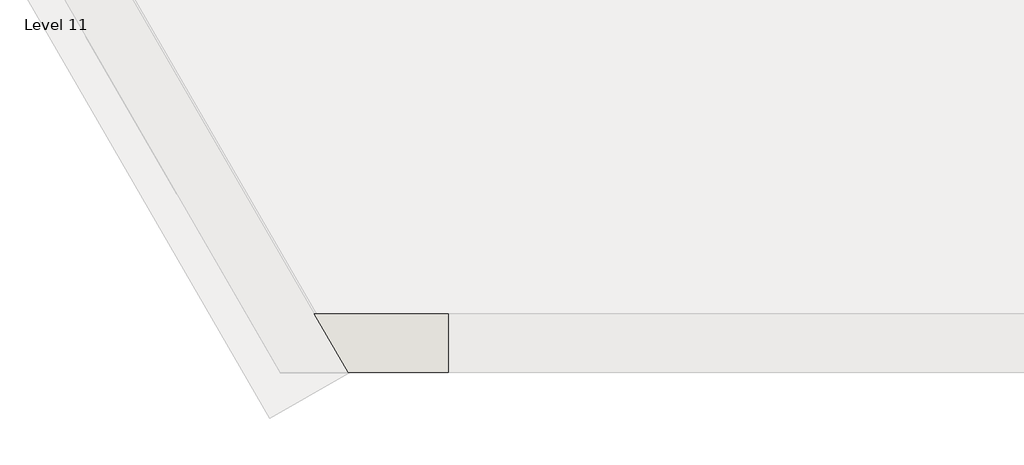
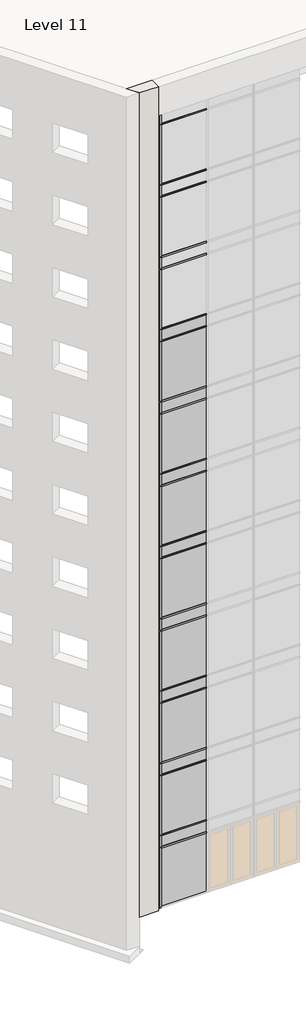
# One storey, part 1 of 6: 89 members, 38 plates, 1 wall.
# Revit data of these elements (continued)
# Type "Rectangular Mullion : 50x150mm" (continued)
#   built-in parameter 1007301 = 0.082021 (stored number, unit not read)
#   built-in parameter 1007300 = 0.082021 (stored number, unit not read)
# Type "System Panel : Glazed"
#   Keynote = "H11"
#   Construction Type Id = "GSP4R"
#   Analytic Construction = "1/8 in Pilkington single glazing"
#   Visual Light Transmittance = 0.9
#   Solar Heat Gain Coefficient = 0.86
#   Heat Transfer Coefficient (U) = 6.7069 W/(m²·K)
# Type "Wall-Ext_102Bwk-40AIR_65Ins-215LBlk-15P"
#   Keynote = "F10"
#   Layers, outside or top first: 102.5 mm "Brick, Common, Brown" (function 4); 40 mm "Air" (function 3); 65 mm "Rigid insulation" (function 3); 215 mm "Concrete Masonry Units _Low Density" (function 1); 15 mm "Plaster" (function 5)
# Elements 1, 2, 3, 4, 5, 6, 7, 8, 9, 10, 11, 12, 13, 14, 15, 16, 17, 18, 19, 20, 21, 22, 23, 24, 25, 26, 27, 28, 29, 30, 31, 32, 33, 34, 35, 36, 37, 38, 39, 40, 41, 42, 43, 44, 45, 46, 47, 48, 49, 50, 51, 52, 53, 54, 55, 56, 57, 58, 59, 60, 61, 62, 63, 64, 65, 66, 67, 68, 69, 70, 71, 72, 73, 74, 75, 76, 77, 78, 79, 80, 81, 82, 83, 84, 85, 86, 87, 88, 89 (IfcMember, "Rectangular Mullion : 50x150mm")
#   Phase Created = New Construction
#   Materials on its faces: "Aluminium"
# Elements 90, 91, 92, 93, 94, 95, 96, 97, 98, 99, 100, 101, 102, 103, 104, 105, 106, 107, 108, 109, 110, 111, 112, 113, 114, 115, 116, 117, 118, 119, 120, 121, 122, 123, 124, 125, 126, 127 (IfcPlate, "System Panel : Glazed")
#   Phase Created = New Construction
#   Materials on its faces: "Glass"
# Element 128 (IfcWall, "Wall-Ext_102Bwk-40AIR_65Ins-215LBlk-15P")
#   built-in parameter 1001111 = -33000 mm
#   Top Offset = 0 mm
#   Base Offset = -33000 mm
#   Unconnected Height = 34200 mm
#   wall height = 34200 mm
#   Phase Created = New Construction
#   Base Constraint = Level 11
#   Materials on its faces: "Default Wall", "Plaster", "Brick, Common, Brown"
# Materials
#   "Brick, Common, Brown": class "Masonry", colour RGB 120 120 120, transparency 0, Description = "Common brick, brown", Cost = 0
#   "Air": class "Gas", colour RGB 255 255 255, transparency 0, Description = "Air", Cost = 0
#   "Rigid insulation": class "Generic", colour RGB 127 127 127, transparency 0, Description = "Rigid foam insulation board", Cost = 0
#   "Concrete Masonry Units _Low Density": class "Masonry", colour RGB 181 181 181, transparency 0, Description = "Concrete masonry units", Cost = 0
#   "Plaster": class "Generic", colour RGB 249 249 249, transparency 0, Description = "Plaster", Cost = 0
#   "Aluminium": class "Metal", colour RGB 247 247 247, transparency 0, Description = "Aluminium 6061", Cost = 0
#   "Glass": class "Glass", colour RGB 0 128 192, transparency 0.9, Description = "Soda Lime Glass", Cost = 0
#   "Default Wall": class "Miscellaneous", colour RGB 128 128 128, transparency 0, Comments = "Rendering appearance not upgraded "
